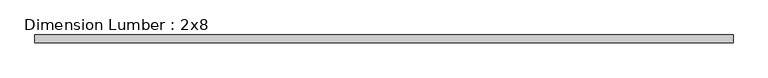
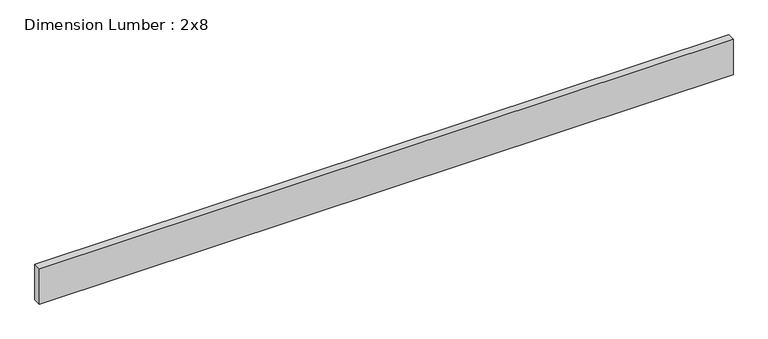
"""IFC4 building model written with IfcOpenShell, lengths in millimetres: beam geometry, Dimension Lumber : 2x8."""

from ifc_helpers import new_model, si_unit, frame, origin, place, context, project, spatial, polyline, outline, extrude, source, transform, mapped, element, save


def dimension_lumber_2x8_2ba21861(model_context):
    return source(origin(), model_context, "Body", "SweptSolid", [
        extrude(outline(polyline([(2227.6894756, 19.05), (2227.6894756, -19.05), (-1175.9105244, -19.05), (-1175.9105244, 19.05), (2227.6894756, 19.05)])), frame((0.0, 0.0, -92.075), z_axis=(0.0, 0.0, 1.0), x_axis=(1.0, 0.0, 0.0)), (0.0, 0.0, 1.0), 184.15),
    ])


if __name__ == "__main__":
    model = new_model("IFC4")
    model_context = context("Model", 3, world=origin())
    ifc_project = project(units=[si_unit("LENGTHUNIT", "METRE", prefix="MILLI")], contexts=[model_context])
    site = spatial("IfcSite", under=ifc_project)
    building = spatial("IfcBuilding", under=site)
    placement = place(None, origin())
    dimension_lumber_2x8_shape = dimension_lumber_2x8_2ba21861(model_context)
    element("IfcBeam", 1, ObjectType="Dimension Lumber : 2x8", at=placement, inside=building, context=model_context, shape_type="MappedRepresentation", body=[
        mapped(dimension_lumber_2x8_shape, transform((0.0, 0.0, 0.0), x_axis=(1.0, 0.0, 0.0), y_axis=(0.0, 1.0, 0.0), z_axis=(0.0, 0.0, 1.0))),
    ])
    save(model, "model.ifc")

# Revit data of these elements
# Type "Dimension Lumber : 2x8"
#   Assembly Code = "B10"
#   A = 0.0755556 SF
#   Length [instance default] = 5' - 0"
#   b = 0' - 1 1/2"
#   d = 0' - 7 1/4"
#   Structural Material [instance default] = PRE-ENGINEERED TRUSS @ 24" O.C.
# Element 1 (IfcBeam, "Dimension Lumber : 2x8")
#   Structural Material = 2 X 8 FIELD FRAMED PURLINS
#   Materials on its faces: "2 X 8 FIELD FRAMED PURLINS"
# Materials
#   "PRE-ENGINEERED TRUSS @ 24\" O.C.": class "Wood", colour RGB 255 255 255, transparency 0, Description = "Pinus Echinata", Cost = 0
#   "2 X 8 FIELD FRAMED PURLINS": class "Wood", colour RGB 234 198 147, transparency 0, Description = "Pinus Echinata", Cost = 0
